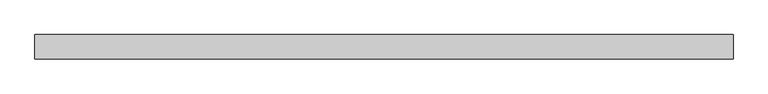
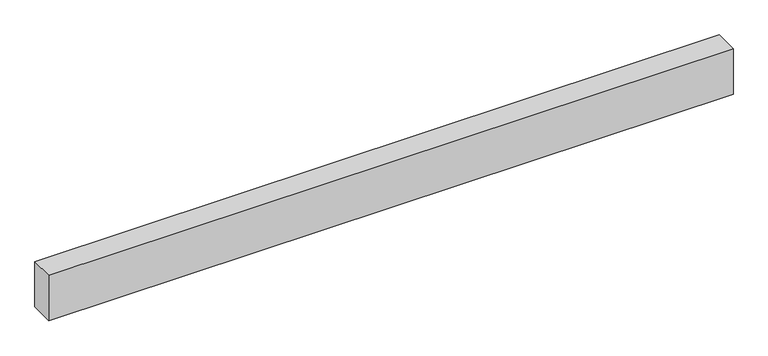
"""IFC4 building model written with IfcOpenShell, lengths in millimetres: beam geometry, Madeira de lei : Berço 6x12cm."""

from ifc_helpers import new_model, si_unit, frame, origin, place, context, project, spatial, polyline, outline, extrude, source, transform, mapped, element, save


def beam_739eac5c(model_context):
    return source(origin(), model_context, "Body", "SweptSolid", [
        extrude(outline(polyline([(854.9999994, 30.0), (854.9999994, -30.0), (-855.0, -30.0), (-855.0, 30.0), (854.9999994, 30.0)])), frame((0.0, 0.0, -60.0), z_axis=(0.0, 0.0, 1.0), x_axis=(1.0, 0.0, 0.0)), (0.0, 0.0, 1.0), 120.0),
    ])


if __name__ == "__main__":
    model = new_model("IFC4")
    model_context = context("Model", 3, world=origin())
    ifc_project = project(units=[si_unit("LENGTHUNIT", "METRE", prefix="MILLI")], contexts=[model_context])
    site = spatial("IfcSite", under=ifc_project)
    building = spatial("IfcBuilding", under=site)
    placement = place(None, origin())
    beam_shape = beam_739eac5c(model_context)
    element("IfcBeam", 1, ObjectType="Madeira de lei : Berço 6x12cm", at=placement, inside=building, context=model_context, shape_type="MappedRepresentation", body=[
        mapped(beam_shape, transform((0.0, 0.0, 0.0), x_axis=(1.0, 0.0, 0.0), y_axis=(0.0, 1.0, 0.0), z_axis=(0.0, 0.0, 1.0))),
    ])
    save(model, "model.ifc")

# Revit data of these elements
# Type "Madeira de lei : Berço 6x12cm"
#   A = 0.02 m²
#   Length [instance default] = 1.524 m
#   b = 0.06 m
#   d = 0.12 m
#   Structural Material [instance default] = none
#   Assembly Code = ""
# Element 1 (IfcBeam, "Madeira de lei : Berço 6x12cm")
#   Structural Material = .MADEIRAMENTO
#   Materials on its faces: ".MADEIRAMENTO"
# Materials
#   ".MADEIRAMENTO": class ".CC_MADEIRAS", colour RGB 212 179 113, transparency 0, Cost = 0
